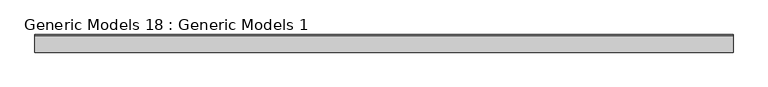
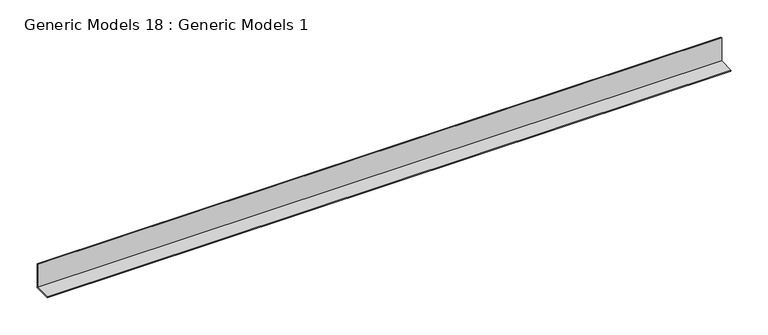
"""IFC4 building model written with IfcOpenShell, lengths in millimetres: proxy geometry, Generic Models 18 : Generic Models 1."""

import ifcopenshell
import ifcopenshell.guid

model = None  # the IFC model being written
_history = None  # IfcOwnerHistory: only IFC2X3 demands one
_inside = {}  # id of a spatial element -> (the spatial element, [elements in it])
_under = {}  # id of a project, library or spatial element -> (it, [spatial elements below it])
_declared = {}  # id of a project -> (the project, [libraries it declares])
_typed = {}  # id of a type object -> (the type object, [elements of that type])
_made_of = {}  # id of a material, layer set ... -> (it, [elements and type objects made of it])


def new_model(schema):
    """Start an empty IFC model of exactly this schema.

    Asked for "IFC4X3", IfcOpenShell would pick the latest addendum, in which some entities
    have other attributes; the version numbers below select the first issue.
    IFC2X3 requires an IfcOwnerHistory on every rooted entity: one is made here for all.
    """
    global model, _history
    if schema == "IFC4X3":
        model = ifcopenshell.file(schema_version=(4, 3, 0, 0))
    else:
        model = ifcopenshell.file(schema=schema)
    _inside.clear()
    _under.clear()
    _declared.clear()
    _typed.clear()
    _made_of.clear()
    _history = None
    if model.schema == "IFC2X3":
        org = make("IfcOrganization", Name="unknown")
        user = make(
            "IfcPersonAndOrganization",
            ThePerson=make("IfcPerson", FamilyName="unknown"),
            TheOrganization=org,
        )
        app = make(
            "IfcApplication",
            ApplicationDeveloper=org,
            Version="unknown",
            ApplicationFullName="unknown",
            ApplicationIdentifier="unknown",
        )
        _history = make(
            "IfcOwnerHistory",
            OwningUser=user,
            OwningApplication=app,
            ChangeAction="ADDED",
            CreationDate=0,
        )
    return model


def make(cls, **values):
    """One entity of the class cls with the attributes given. An attribute that is None is left unset."""
    return model.create_entity(
        cls, **{name: value for name, value in values.items() if value is not None}
    )


def rooted(cls, **values):
    """An entity with a GlobalId (a new one), such as an element, a storey or a relation."""
    return make(cls, GlobalId=ifcopenshell.guid.new(), OwnerHistory=_history, **values)


def si_unit(unit_type, name, prefix=None):
    """IfcSIUnit, for example si_unit("LENGTHUNIT", "METRE", prefix="MILLI")."""
    return make("IfcSIUnit", UnitType=unit_type, Prefix=prefix, Name=name)


def assignment(units):
    """IfcUnitAssignment: the units of a project."""
    return None if units is None else make("IfcUnitAssignment", Units=units)


def point(xyz):
    """IfcCartesianPoint."""
    return None if xyz is None else make("IfcCartesianPoint", Coordinates=xyz)


def direction(xyz):
    """IfcDirection."""
    return None if xyz is None else make("IfcDirection", DirectionRatios=xyz)


def frame(location, z_axis=None, x_axis=None):
    """IfcAxis2Placement3D, a coordinate frame: its origin and axes. An axis left out is left unset."""
    return make(
        "IfcAxis2Placement3D",
        Location=point(location),
        Axis=direction(z_axis),
        RefDirection=direction(x_axis),
    )


def origin():
    """The frame at (0, 0, 0) with its axes left unset."""
    return frame((0.0, 0.0, 0.0))


def place(relative_to, where):
    """IfcLocalPlacement: puts the frame where relative to a parent placement (None: the world)."""
    return make(
        "IfcLocalPlacement", PlacementRelTo=relative_to, RelativePlacement=where
    )


def context(
    kind, dimensions, precision=None, world=None, true_north=None, identifier=None
):
    """IfcGeometricRepresentationContext, for example the 3D "Model" context."""
    return make(
        "IfcGeometricRepresentationContext",
        ContextIdentifier=identifier,
        ContextType=kind,
        CoordinateSpaceDimension=dimensions,
        Precision=precision,
        WorldCoordinateSystem=world,
        TrueNorth=true_north,
    )


def project(units=None, contexts=None):
    """IfcProject with its units and contexts."""
    return rooted(
        "IfcProject",
        Name="project",
        RepresentationContexts=contexts,
        UnitsInContext=assignment(units),
    )


def spatial(cls, under=None, at=None, **own):
    """A site, building, storey or space (cls), placed at a placement, below another one or the project."""
    s = rooted(cls, ObjectPlacement=at, **own)
    if under is not None:
        _under.setdefault(under.id(), (under, []))[1].append(s)
    return s


def polyline(points):
    """IfcPolyline through the points."""
    return make("IfcPolyline", Points=[point(p) for p in points])


def outline(outer, holes=None, kind="AREA"):
    """IfcArbitraryClosedProfileDef: a profile drawn as a closed curve; with holes, ...WithVoids."""
    if holes is None:
        return make("IfcArbitraryClosedProfileDef", ProfileType=kind, OuterCurve=outer)
    return make(
        "IfcArbitraryProfileDefWithVoids",
        ProfileType=kind,
        OuterCurve=outer,
        InnerCurves=holes,
    )


def extrude(swept, where, along, depth):
    """IfcExtrudedAreaSolid: the profile swept, set in the frame where, extruded along a direction by depth."""
    return make(
        "IfcExtrudedAreaSolid",
        SweptArea=swept,
        Position=where,
        ExtrudedDirection=direction(along),
        Depth=depth,
    )


def shape(context_of_items, identifier, shape_type, items):
    """IfcShapeRepresentation: the items that make up one representation, for example the "Body"."""
    return make(
        "IfcShapeRepresentation",
        ContextOfItems=context_of_items,
        RepresentationIdentifier=identifier,
        RepresentationType=shape_type,
        Items=items,
    )


def source(mapping_origin, context_of_items, identifier, shape_type, items):
    """IfcRepresentationMap: a shape defined once, which mapped items show again and again."""
    return make(
        "IfcRepresentationMap",
        MappingOrigin=mapping_origin,
        MappedRepresentation=shape(context_of_items, identifier, shape_type, items),
    )


def transform(
    local_origin,
    x_axis=None,
    y_axis=None,
    z_axis=None,
    scale=None,
    scale2=None,
    scale3=None,
    uniform=True,
):
    """IfcCartesianTransformationOperator3D, or its non-uniform kind. x_axis, y_axis, z_axis: its Axis1, 2, 3."""
    if uniform:
        return make(
            "IfcCartesianTransformationOperator3D",
            Axis1=direction(x_axis),
            Axis2=direction(y_axis),
            LocalOrigin=point(local_origin),
            Scale=scale,
            Axis3=direction(z_axis),
        )
    return make(
        "IfcCartesianTransformationOperator3DnonUniform",
        Axis1=direction(x_axis),
        Axis2=direction(y_axis),
        LocalOrigin=point(local_origin),
        Scale=scale,
        Axis3=direction(z_axis),
        Scale2=scale2,
        Scale3=scale3,
    )


def mapped(mapping_source, mapping_target):
    """IfcMappedItem: shows the shape of a source again, moved by a transform."""
    return make(
        "IfcMappedItem", MappingSource=mapping_source, MappingTarget=mapping_target
    )


def made_of(thing, what):
    """Note that an element or type object is made of a material, layer set ...; save() writes the relation."""
    if what is not None:
        _made_of.setdefault(what.id(), (what, []))[1].append(thing)
    return thing


def element(
    cls,
    number,
    at=None,
    inside=None,
    cuts=None,
    type_object=None,
    material=None,
    context=None,
    identifier="Body",
    shape_type=None,
    held_by="IfcProductDefinitionShape",
    body=None,
    shapes=None,
    **own,
):
    """One element of the class cls, such as IfcWall. Its Tag is "e" and its number.

    at: its placement. inside: the storey or other place that contains it. cuts: it is an
    opening in that element (IfcRelVoidsElement). A single representation is given by context,
    identifier, shape_type and body (its items); several are given by shapes. held_by: the class
    of the entity that holds the representations. save() writes the other relations.
    """
    e = rooted(cls, Tag="e%d" % number, ObjectPlacement=at, **own)
    if body is not None:
        shapes = [shape(context, identifier, shape_type, body)]
    if shapes is not None:
        e.Representation = make(held_by, Representations=shapes)
    if inside is not None:
        _inside.setdefault(inside.id(), (inside, []))[1].append(e)
    if cuts is not None:
        rooted(
            "IfcRelVoidsElement", RelatingBuildingElement=cuts, RelatedOpeningElement=e
        )
    if type_object is not None:
        _typed.setdefault(type_object.id(), (type_object, []))[1].append(e)
    return made_of(e, material)


def aggregate(whole, parts):
    """IfcRelAggregates: a whole, such as a stair, and the parts it consists of."""
    return rooted("IfcRelAggregates", RelatingObject=whole, RelatedObjects=parts)


def save(model, path):
    """Write the relations noted so far, then the file.

    IfcRelAggregates (storeys below a building ...), IfcRelContainedInSpatialStructure (elements
    in a storey), IfcRelDefinesByType, IfcRelAssociatesMaterial and IfcRelDeclares: one each for
    every whole, place, type object, material and project.
    """
    for whole, parts in _under.values():
        aggregate(whole, parts)
    for where, things in _inside.values():
        rooted(
            "IfcRelContainedInSpatialStructure",
            RelatedElements=things,
            RelatingStructure=where,
        )
    for kind, things in _typed.values():
        rooted("IfcRelDefinesByType", RelatedObjects=things, RelatingType=kind)
    for what, things in _made_of.values():
        rooted("IfcRelAssociatesMaterial", RelatedObjects=things, RelatingMaterial=what)
    for by, libraries in _declared.values():
        rooted("IfcRelDeclares", RelatingContext=by, RelatedDefinitions=libraries)
    model.write(path)


def generic_models_18_generic_models_1_e87dc61f(model_context):
    return source(origin(), model_context, "Body", "SweptSolid", [
        extrude(outline(polyline([(39419.9928995, 2654.3), (39419.9928995, 2614.6125), (39393.0053995, 2614.6125), (39393.0053995, 2616.2), (39418.4053995, 2616.2), (39418.4053995, 2654.3), (39419.9928995, 2654.3)])), frame((51512.0577305, 0.0, 0.0), z_axis=(1.0, 0.0, 0.0), x_axis=(0.0, 1.0, 0.0)), (0.0, 0.0, 1.0), 1066.8),
    ])


if __name__ == "__main__":
    model = new_model("IFC4")
    model_context = context("Model", 3, world=origin())
    ifc_project = project(units=[si_unit("LENGTHUNIT", "METRE", prefix="MILLI")], contexts=[model_context])
    site = spatial("IfcSite", under=ifc_project)
    building = spatial("IfcBuilding", under=site)
    placement = place(None, origin())
    generic_models_18_generic_models_1_shape = generic_models_18_generic_models_1_e87dc61f(model_context)
    element("IfcBuildingElementProxy", 1, Name="Generic Models 18 : Generic Models 1", ObjectType="Generic Models 18 : Generic Models 1", at=placement, inside=building, context=model_context, shape_type="MappedRepresentation", body=[
        mapped(generic_models_18_generic_models_1_shape, transform((0.0, 0.0, 0.0), x_axis=(1.0, 0.0, 0.0), y_axis=(0.0, 1.0, 0.0), z_axis=(0.0, 0.0, 1.0))),
    ])
    save(model, "model.ifc")

# Revit data of these elements
# Element 1 (IfcBuildingElementProxy, "Generic Models 18 : Generic Models 1")
#   Materials on its faces: "ACOUSTICAL PERMITER TRACK TO MATCH EXISTING"
# Materials
#   "ACOUSTICAL PERMITER TRACK TO MATCH EXISTING": class "Generic", colour RGB 120 120 120, transparency 0, Cost = 0
